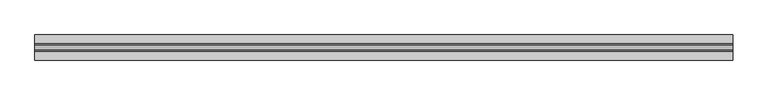
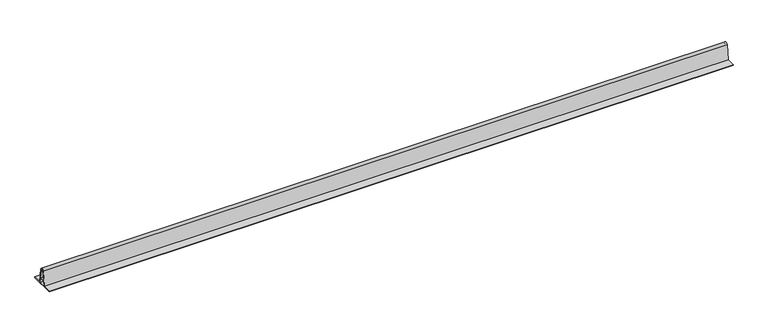
"""IFC4 building model written with IfcOpenShell, lengths in millimetres: proxy geometry, TN_А-профиль, серый : А-профиль h50 (2 м), серый."""

from ifc_helpers import new_model, si_unit, point, frame, frame_2d, origin, place, context, project, spatial, polyline, circle_curve, trimmed, segment, composite_curve, outline, extrude, source, transform, mapped, element, save


def specialty_equipment_a3cd9701(model_context):
    return source(origin(), model_context, "Body", "SweptSolid", [
        extrude(outline(composite_curve([segment(polyline([(36.0, 0.0), (-36.0, 0.0), (-36.0, 2.0), (-12.0, 2.0), (-5.9408737, 44.8402496)]), True, "CONTINUOUS"), segment(trimmed(circle_curve(frame_2d((0.0, 44.0)), 6.0), [point((-5.9408737, 44.8402496))], [point((5.9408737, 44.8402496))], False, "CARTESIAN"), True, "CONTINUOUS"), segment(polyline([(5.9408737, 44.8402496), (12.0, 2.0), (36.0, 2.0), (36.0, 0.0)]), True, "CONTINUOUS")], self_intersect=False), holes=[composite_curve([segment(polyline([(-5.8386597, 17.0), (5.8386597, 17.0), (1.9802912, 44.2800832)]), True, "CONTINUOUS"), segment(trimmed(circle_curve(frame_2d((0.0, 44.0)), 2.0), [point((1.9802912, 44.2800832))], [point((-1.9802912, 44.2800832))], True, "CARTESIAN"), True, "CONTINUOUS"), segment(polyline([(-1.9802912, 44.2800832), (-5.8386597, 17.0)]), True, "CONTINUOUS")], self_intersect=False), polyline([(6.2629658, 14.0), (-6.2629658, 14.0), (-7.9601902, 2.0), (7.9601902, 2.0), (6.2629658, 14.0)])]), frame((0.0, 0.0, 0.0), z_axis=(1.0, 0.0, 0.0), x_axis=(0.0, 1.0, 0.0)), (0.0, 0.0, 1.0), 2000.0),
    ])


if __name__ == "__main__":
    model = new_model("IFC4")
    model_context = context("Model", 3, world=origin())
    ifc_project = project(units=[si_unit("LENGTHUNIT", "METRE", prefix="MILLI")], contexts=[model_context])
    site = spatial("IfcSite", under=ifc_project)
    building = spatial("IfcBuilding", under=site)
    placement = place(None, origin())
    specialty_equipment_shape = specialty_equipment_a3cd9701(model_context)
    element("IfcBuildingElementProxy", 1, Name="TN_А-профиль, серый : А-профиль h50 (2 м), серый", ObjectType="TN_А-профиль, серый : А-профиль h50 (2 м), серый", at=placement, inside=building, context=model_context, shape_type="MappedRepresentation", body=[
        mapped(specialty_equipment_shape, transform((0.0, 0.0, 0.0), x_axis=(1.0, 0.0, 0.0), y_axis=(0.0, 1.0, 0.0), z_axis=(0.0, 0.0, 1.0))),
    ])
    save(model, "model.ifc")

# Revit data of these elements
# Type "TN_А-профиль, серый : А-профиль h50 (2 м), серый"
#   Description = "А-профиль изготавливается из высококачественного поливинилхлорида, устойчивого к атмосферному воздействию и ультрафиолетовому излучению. Применяется совместно с ПВХ мембранами ТехноНИКОЛЬ. Приваривается к мембране гомогенно при помощи горячего воздуха."
#   Type Comments = "п.м."
#   Manufacturer = "ТехноНИКОЛЬ"
#   URL = "https://nav.tn.ru/catalog/krovlya/komplektatsiya-dlya-krovli/a-profil-iz-pvkh/?sphrase_id=266377"
#   ADSK_Примечание = ""
#   ADSK_Обозначение [instance default] = "ТехноНИКОЛЬ"
#   ADSK_Наименование = "А-профиль h50 (2 м), серый"
#   ADSK_Масса_Текст = ""
#   ADSK_Марка = ""
#   ADSK_Код изделия = "634765"
#   ADSK_Завод-изготовитель [instance default] = "ТехноНИКОЛЬ"
#   ADSK_Единица измерения [instance default] = "п.м."
#   ADSK_Группирование = "Комплектующие и воронки"
#   ADSK_URL страницы изделия = "https://nav.tn.ru/catalog/krovlya/komplektatsiya-dlya-krovli/a-profil-iz-pvkh/?sphrase_id=266377"
#   ADSK_URL документации изделия = "https://nav.tn.ru/upload/iblock/7bd/Tekhlist-7.58_A_profil_rus.pdf"
#   built-in parameter 1001306 [instance default] = 3.28084 (stored number, unit not read)
#   ADSK_Размер_Длина [instance default] = 1000 mm
#   ADSK_Количество [instance default] = 1
#   Видимость_Тип профиля 50 = yes
#   Видимость_Тип профиля 25 = no
#   Материал = TN_ПВХ_Серый
#   Default Elevation = 0
# Element 1 (IfcBuildingElementProxy, "TN_А-профиль, серый : А-профиль h50 (2 м), серый")
#   built-in parameter 1001306 = 6.56168 (stored number, unit not read)
#   ADSK_Размер_Длина = 2000 mm
#   ADSK_Количество = 2
#   Materials on its faces: "TN_ПВХ_Серый"
# Materials
#   "TN_ПВХ_Серый": class "Типовые", colour RGB 192 192 192, transparency 0, Cost = 0
